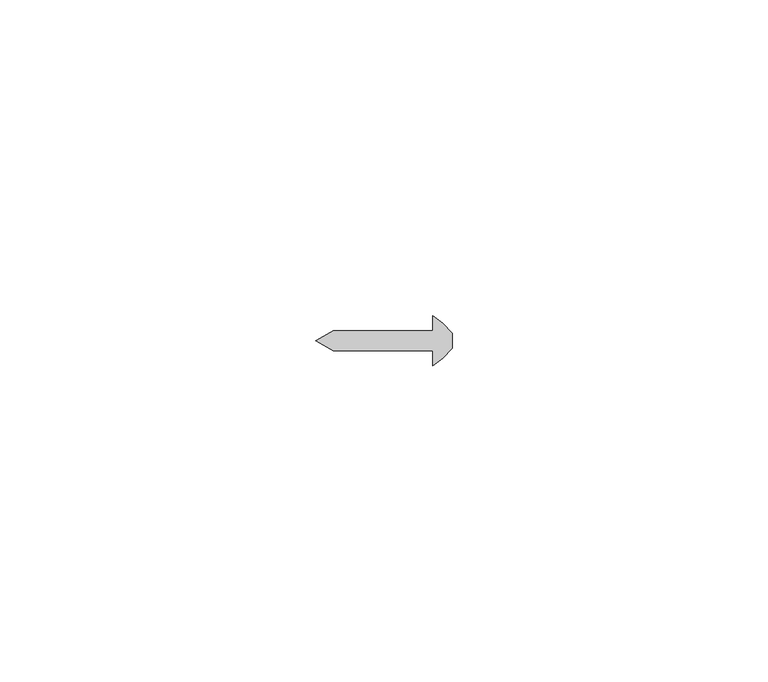
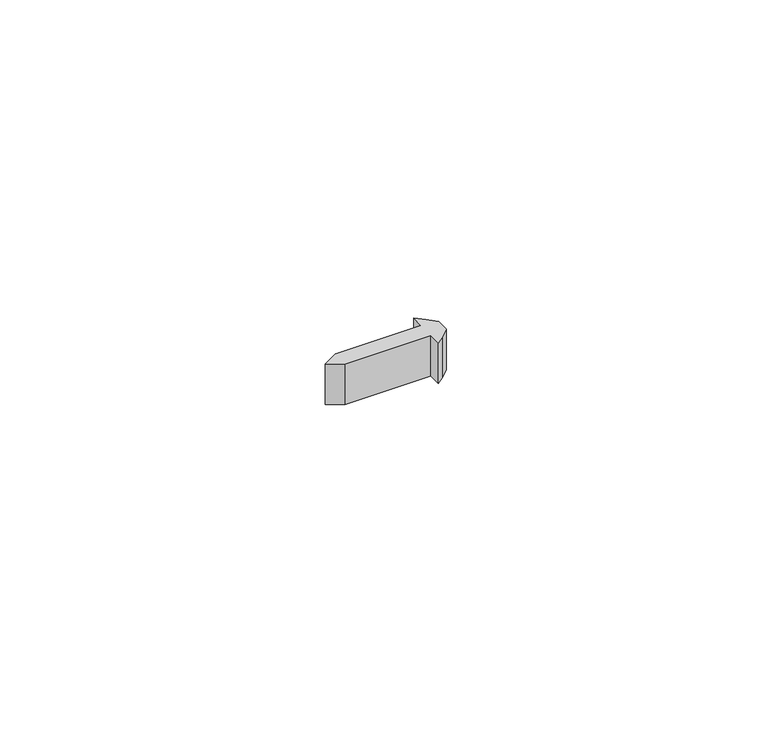
"""IFC4 building model written with IfcOpenShell, lengths in millimetres: proxy geometry, Generic Models 7:Generic Models 1:3:Generic Models 1:3 : Generic Models 7:Generic Models 1:305549:3:Generic Models 1:3:Generic Models 1:3 : Generic Models 7:Generic Models 1:305549:3 : Generic Models 7:Generic Models 1:3:Generic Models 1:3 : Generic Models 7:Generic Models 1:305549:301244:12 : Generic Models 7:Generic Models 1:3:Generic Models 1:3 : Generic Models 7:Generic Models 1:305549:3:Generic Models 1:3:Generic Models 1:3 : Generic Models 7:Generic Models 1:305549:3 : Generic Models 7:Generic Models 1:3:Generic Models 1:3 : Generic Models 7:Generic Models 1:305549:301244:308848."""

from ifc_helpers import new_model, si_unit, frame, origin, place, context, project, spatial, polyline, outline, extrude, source, transform, mapped, element, save


def generic_models_370d4224(model_context):
    return source(origin(), model_context, "Body", "SweptSolid", [
        extrude(outline(polyline([(579391.8492239, -578999.1038841), (579391.8492239, -578996.7226341), (579393.3762819, -578997.9408297), (579394.9281721, -578999.4927199), (579394.9281721, -579001.8900483), (579393.3762819, -579003.4419385), (579391.8492239, -579004.6601341), (579391.8492239, -579002.2788841), (579376.0399684, -579002.2788841), (579373.2903378, -579000.6913841), (579376.0399684, -578999.1038841), (579391.8492239, -578999.1038841)])), frame((0.0, 0.0, 4907.75625), z_axis=(0.0, 0.0, 1.0), x_axis=(1.0, 0.0, 0.0)), (0.0, 0.0, 1.0), 7.9375),
    ])


if __name__ == "__main__":
    model = new_model("IFC4")
    model_context = context("Model", 3, world=origin())
    ifc_project = project(units=[si_unit("LENGTHUNIT", "METRE", prefix="MILLI")], contexts=[model_context])
    site = spatial("IfcSite", under=ifc_project)
    building = spatial("IfcBuilding", under=site)
    placement = place(None, origin())
    generic_models_shape = generic_models_370d4224(model_context)
    element("IfcBuildingElementProxy", 1, Name="Generic Models 7:Generic Models 1:3:Generic Models 1:3 : Generic Models 7:Generic Models 1:305549:3:Generic Models 1:3:Generic Models 1:3 : Generic Models 7:Generic Models 1:305549:3 : Generic Models 7:Generic Models 1:3:Generic Models 1:3 : Generic Models 7:Generic Models 1:305549:301244:12 : Generic Models 7:Generic Models 1:3:Generic Models 1:3 : Generic Models 7:Generic Models 1:305549:3:Generic Models 1:3:Generic Models 1:3 : Generic Models 7:Generic Models 1:305549:3 : Generic Models 7:Generic Models 1:3:Generic Models 1:3 : Generic Models 7:Generic Models 1:305549:301244:308848", ObjectType="Generic Models 7:Generic Models 1:3:Generic Models 1:3 : Generic Models 7:Generic Models 1:305549:3:Generic Models 1:3:Generic Models 1:3 : Generic Models 7:Generic Models 1:305549:3 : Generic Models 7:Generic Models 1:3:Generic Models 1:3 : Generic Models 7:Generic Models 1:305549:301244:12 : Generic Models 7:Generic Models 1:3:Generic Models 1:3 : Generic Models 7:Generic Models 1:305549:3:Generic Models 1:3:Generic Models 1:3 : Generic Models 7:Generic Models 1:305549:3 : Generic Models 7:Generic Models 1:3:Generic Models 1:3 : Generic Models 7:Generic Models 1:305549:301244:308848", at=placement, inside=building, context=model_context, shape_type="MappedRepresentation", body=[
        mapped(generic_models_shape, transform((0.0, 0.0, 0.0), x_axis=(1.0, 0.0, 0.0), y_axis=(0.0, 1.0, 0.0), z_axis=(0.0, 0.0, 1.0))),
    ])
    save(model, "model.ifc")

# Revit data of these elements
# Type "Generic Models 7:Generic Models 1:3:Generic Models 1:3 : Generic Models 7:Generic Models 1:305549:3:Generic Models 1:3:Generic Models 1:3 : Generic Models 7:Generic Models 1:305549:3 : Generic Models 7:Generic Models 1:3:Generic Models 1:3 : Generic Models 7:Generic Models 1:305549:301244:12 : Generic Models 7:Generic Models 1:3:Generic Models 1:3 : Generic Models 7:Generic Models 1:305549:3:Generic Models 1:3:Generic Models 1:3 : Generic Models 7:Generic Models 1:305549:3 : Generic Models 7:Generic Models 1:3:Generic Models 1:3 : Generic Models 7:Generic Models 1:305549:301244:308848"
#   NameOverride = "Generic Models 7:Generic Models 1:3:Generic Models 1:3 : Generic Models 7:Generic Models 1:305549:3:Generic Models 1:3:Generic Models 1:3 : Generic Models 7:Generic Models 1:305549:3 : Generic Models 7:Generic Models 1:3:Generic Models 1:3 : Generic Models 7:Generic Models 1:305549:301244:308848"
#   ObjectTypeOverride = "Generic Models 1:3:Generic Models 1:3 : Generic Models 7:Generic Models 1:305549:3 : Generic Models 7:Generic Models 1:3:Generic Models 1:3 : Generic Models 7:Generic Models 1:305549:301244"
#   Reference = "Generic Models 1"
#   Tag = "308848"
# Element 1 (IfcBuildingElementProxy, "Generic Models 7:Generic Models 1:3:Generic Models 1:3 : Generic Models 7:Generic Models 1:305549:3:Generic Models 1:3:Generic Models 1:3 : Generic Models 7:Generic Models 1:305549:3 : Generic Models 7:Generic Models 1:3:Generic Models 1:3 : Generic Models 7:Generic Models 1:305549:301244:12 : Generic Models 7:Generic Models 1:3:Generic Models 1:3 : Generic Models 7:Generic Models 1:305549:3:Generic Models 1:3:Generic Models 1:3 : Generic Models 7:Generic Models 1:305549:3 : Generic Models 7:Generic Models 1:3:Generic Models 1:3 : Generic Models 7:Generic Models 1:305549:301244:308848")
#   Materials on its faces: "FASTENERS (T.B.D)"
# Materials
#   "FASTENERS (T.B.D)": class "Generic", colour RGB 120 120 120, transparency 0, Cost = 0
